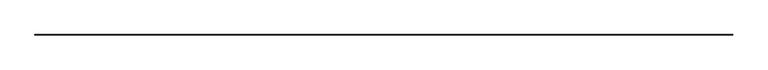
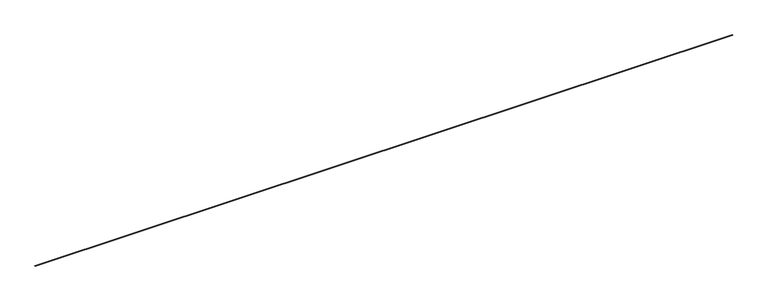
"""IFC4 building model written with IfcOpenShell, lengths in millimetres: proxy geometry, Inner panel:Inner panel:1:Inner panel:1 : Inner panel:Inner panel:300324:2:Inner panel:1:Inner panel:1 : Inner panel:Inner panel:300324:2 : Inner panel:Inner panel:1:Inner panel:1 : Inner panel:Inner panel:300324:300043:42 : Inner panel:Inner panel:1:Inner panel:1 : Inner panel:Inner panel:300324:2:Inner panel:1:Inner panel:1 : Inner panel:Inner panel:300324:2 : Inner panel:Inner panel:1:Inner panel:1 : Inner panel:Inner panel:300324:300043:308120."""

from ifc_helpers import new_model, si_unit, frame, origin, place, context, project, spatial, polyline, outline, extrude, source, transform, mapped, element, save


def generic_models_81b97110(model_context):
    return source(origin(), model_context, "Body", "SweptSolid", [
        extrude(outline(polyline([(-580492.4474374, 3849.6087907), (-580494.0335611, 3887.6757607), (-580455.966591, 3889.2618845), (-580454.3804673, 3851.1949144), (-580492.4474374, 3849.6087907)]), holes=[polyline([(-580490.1673845, 3852.087109), (-580456.8587856, 3853.4749673), (-580458.2466439, 3886.7835661), (-580491.5552427, 3885.3957078), (-580490.1673845, 3852.087109)])]), frame((579104.5117239, 0.0, 0.0), z_axis=(1.0, 0.0, 0.0), x_axis=(0.0, 1.0, 0.0)), (0.0, 0.0, 1.0), 88442.8),
    ])


if __name__ == "__main__":
    model = new_model("IFC4")
    model_context = context("Model", 3, world=origin())
    ifc_project = project(units=[si_unit("LENGTHUNIT", "METRE", prefix="MILLI")], contexts=[model_context])
    site = spatial("IfcSite", under=ifc_project)
    building = spatial("IfcBuilding", under=site)
    placement = place(None, origin())
    generic_models_shape = generic_models_81b97110(model_context)
    element("IfcBuildingElementProxy", 1, Name="Inner panel:Inner panel:1:Inner panel:1 : Inner panel:Inner panel:300324:2:Inner panel:1:Inner panel:1 : Inner panel:Inner panel:300324:2 : Inner panel:Inner panel:1:Inner panel:1 : Inner panel:Inner panel:300324:300043:42 : Inner panel:Inner panel:1:Inner panel:1 : Inner panel:Inner panel:300324:2:Inner panel:1:Inner panel:1 : Inner panel:Inner panel:300324:2 : Inner panel:Inner panel:1:Inner panel:1 : Inner panel:Inner panel:300324:300043:308120", ObjectType="Inner panel:Inner panel:1:Inner panel:1 : Inner panel:Inner panel:300324:2:Inner panel:1:Inner panel:1 : Inner panel:Inner panel:300324:2 : Inner panel:Inner panel:1:Inner panel:1 : Inner panel:Inner panel:300324:300043:42 : Inner panel:Inner panel:1:Inner panel:1 : Inner panel:Inner panel:300324:2:Inner panel:1:Inner panel:1 : Inner panel:Inner panel:300324:2 : Inner panel:Inner panel:1:Inner panel:1 : Inner panel:Inner panel:300324:300043:308120", at=placement, inside=building, context=model_context, shape_type="MappedRepresentation", body=[
        mapped(generic_models_shape, transform((0.0, 0.0, 0.0), x_axis=(1.0, 0.0, 0.0), y_axis=(0.0, 1.0, 0.0), z_axis=(0.0, 0.0, 1.0))),
    ])
    save(model, "model.ifc")

# Revit data of these elements
# Type "Inner panel:Inner panel:1:Inner panel:1 : Inner panel:Inner panel:300324:2:Inner panel:1:Inner panel:1 : Inner panel:Inner panel:300324:2 : Inner panel:Inner panel:1:Inner panel:1 : Inner panel:Inner panel:300324:300043:42 : Inner panel:Inner panel:1:Inner panel:1 : Inner panel:Inner panel:300324:2:Inner panel:1:Inner panel:1 : Inner panel:Inner panel:300324:2 : Inner panel:Inner panel:1:Inner panel:1 : Inner panel:Inner panel:300324:300043:308120"
#   NameOverride = "Inner panel:Inner panel:1:Inner panel:1 : Inner panel:Inner panel:300324:2:Inner panel:1:Inner panel:1 : Inner panel:Inner panel:300324:2 : Inner panel:Inner panel:1:Inner panel:1 : Inner panel:Inner panel:300324:300043:308120"
#   ObjectTypeOverride = "Inner panel:1:Inner panel:1 : Inner panel:Inner panel:300324:2 : Inner panel:Inner panel:1:Inner panel:1 : Inner panel:Inner panel:300324:300043"
#   Reference = "Inner panel"
#   Tag = "308120"
# Element 1 (IfcBuildingElementProxy, "Inner panel:Inner panel:1:Inner panel:1 : Inner panel:Inner panel:300324:2:Inner panel:1:Inner panel:1 : Inner panel:Inner panel:300324:2 : Inner panel:Inner panel:1:Inner panel:1 : Inner panel:Inner panel:300324:300043:42 : Inner panel:Inner panel:1:Inner panel:1 : Inner panel:Inner panel:300324:2:Inner panel:1:Inner panel:1 : Inner panel:Inner panel:300324:2 : Inner panel:Inner panel:1:Inner panel:1 : Inner panel:Inner panel:300324:300043:308120")
#   Materials on its faces: "1 1/2\" X 1 1/2\" x 1/8\" ALUM. TUBE (6061-T6) - (2) #16 WOOD SCREWS WITH 2.5\" EMBED AT EACH GLULAM - (1) SCREW AT ENDS"
# Materials
#   "1 1/2\" X 1 1/2\" x 1/8\" ALUM. TUBE (6061-T6) - (2) #16 WOOD SCREWS WITH 2.5\" EMBED AT EACH GLULAM - (1) SCREW AT ENDS": class "Unassigned", colour RGB 202 201 200, transparency 0, Cost = 0
